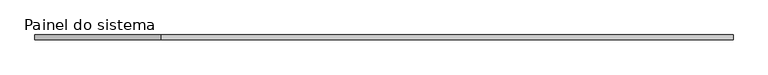
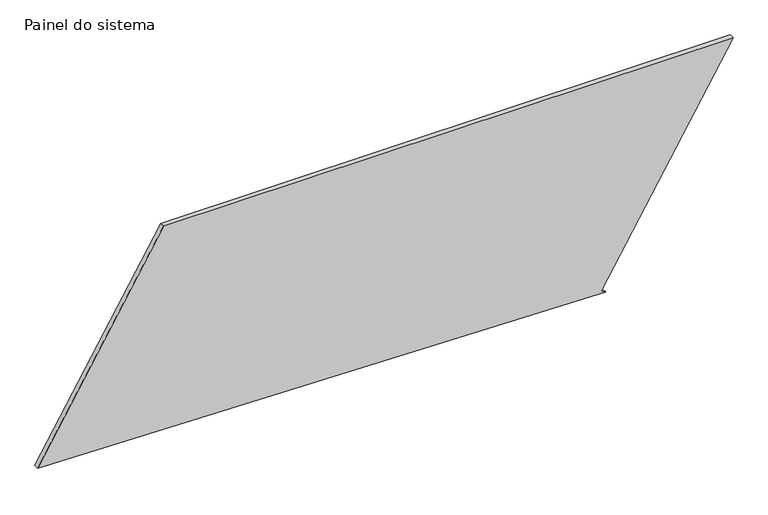
"""IFC4 building model written with IfcOpenShell, lengths in millimetres: plate geometry, Painel do sistema : Envidraçado."""

from ifc_helpers import new_model, si_unit, frame, origin, place, context, project, spatial, polyline, outline, extrude, source, transform, mapped, element, save


def painel_do_sistema_e1affe32(model_context):
    return source(origin(), model_context, "Body", "SweptSolid", [
        extrude(outline(polyline([(0.0, 1144.8011752), (12.7505939, 1123.2971674), (1167.7739494, 1808.1571202), (1167.7739494, -1153.6500112), (63.9409773, -1808.1571202), (0.0, 1144.8011752)])), frame((0.0, 24.5, 0.0), z_axis=(0.0, 1.0, 0.0), x_axis=(0.0, 0.0, 1.0)), (0.0, 0.0, 1.0), 25.0),
    ])


if __name__ == "__main__":
    model = new_model("IFC4")
    model_context = context("Model", 3, world=origin())
    ifc_project = project(units=[si_unit("LENGTHUNIT", "METRE", prefix="MILLI")], contexts=[model_context])
    site = spatial("IfcSite", under=ifc_project)
    building = spatial("IfcBuilding", under=site)
    placement = place(None, origin())
    painel_do_sistema_shape = painel_do_sistema_e1affe32(model_context)
    element("IfcPlate", 1, ObjectType="Painel do sistema : Envidraçado", at=placement, inside=building, context=model_context, shape_type="MappedRepresentation", body=[
        mapped(painel_do_sistema_shape, transform((0.0, 0.0, 0.0), x_axis=(1.0, 0.0, 0.0), y_axis=(0.0, 1.0, 0.0), z_axis=(0.0, 0.0, 1.0))),
    ])
    save(model, "model.ifc")

# Revit data of these elements
# Type "Painel do sistema : Envidraçado"
#   Construction Type Id = "GSP4R"
#   Analytic Construction = "Vidraça única Pilkington 1/8 pol"
#   Visual Light Transmittance = 0.9
#   Solar Heat Gain Coefficient = 0.86
#   Heat Transfer Coefficient (U) = 6.7069 W/(m²·K)
# Element 1 (IfcPlate, "Painel do sistema : Envidraçado")
#   Materials on its faces: "Vidro"
# Materials
#   "Vidro": class "Vidro", colour RGB 0 128 192, transparency 0.9, Description = "Vidro de sílica", Cost = 0
